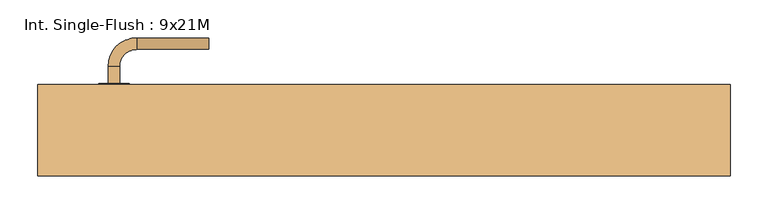
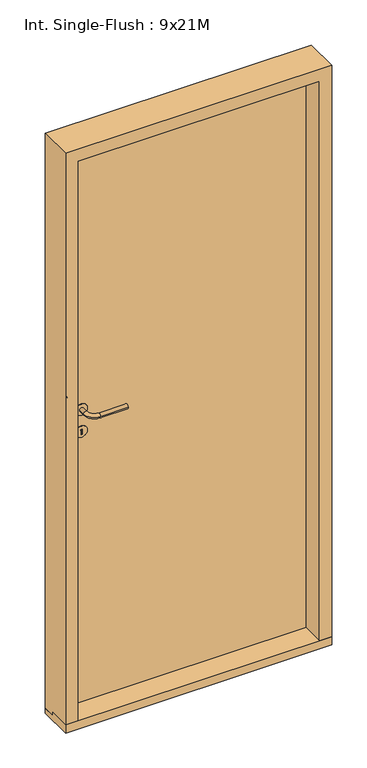
"""IFC4 building model written with IfcOpenShell, lengths in millimetres: door geometry, Int. Single-Flush : 9x21M."""

from ifc_helpers import new_model, si_unit, point, frame, frame_2d, origin, place, context, project, spatial, polyline, circle_curve, ellipse_curve, trimmed, segment, composite_curve, outline, extrude, faceted_brep, source, transform, mapped, element, save
from ifc_brep_helpers import plane_surface, cylinder_surface, revolved_surface, advanced_brep


def int_single_flush_9x21m_be440b31(model_context):
    return source(origin(), model_context, "Body", "SolidModel", [
        extrude(outline(composite_curve([segment(trimmed(circle_curve(frame_2d((1090.0, -356.0)), 20.0), [point((1070.0, -356.0))], [point((1110.0, -356.0))], False, "CARTESIAN"), True, "CONTINUOUS"), segment(trimmed(circle_curve(frame_2d((1090.0, -356.0)), 20.0), [point((1110.0, -356.0))], [point((1070.0, -356.0))], False, "CARTESIAN"), True, "CONTINUOUS")], self_intersect=False)), frame((0.0, 60.0, 0.0), z_axis=(0.0, 1.0, 0.0), x_axis=(0.0, 0.0, 1.0)), (0.0, 0.0, 1.0), 2.0),
        advanced_brep(
        [(-363.5, 62.0, 1090.0), (-348.5, 62.0, 1090.0), (-363.5, 84.5, 1090.0), (-348.5, 84.5, 1090.0), (-326.0, 107.0, 1090.0), (-326.0, 122.0, 1090.0), (-231.0, 122.0, 1090.0), (-231.0, 107.0, 1090.0)],
        [
            (0, 1, circle_curve(frame((-356.0, 62.0, 1090.0), z_axis=(0.0, -1.0, 0.0), x_axis=(1.0, 0.0, 0.0)), 7.5)),
            (1, 0, circle_curve(frame((-356.0, 62.0, 1090.0), z_axis=(0.0, -1.0, 0.0), x_axis=(1.0, 0.0, 0.0)), 7.5)),
            (0, 2),
            (2, 3, circle_curve(frame((-356.0, 84.5, 1090.0), z_axis=(0.0, -1.0, 0.0), x_axis=(1.0, 0.0, 0.0)), 7.5)),
            (3, 1),
            (3, 2, circle_curve(frame((-356.0, 84.5, 1090.0), z_axis=(0.0, -1.0, 0.0), x_axis=(1.0, 0.0, 0.0)), 7.5)),
            (4, 3, circle_curve(frame((-326.0, 84.5, 1090.0), z_axis=(0.0, 0.0, 1.0), x_axis=(-1.0, 0.0, 0.0)), 22.5)),
            (2, 5, circle_curve(frame((-326.0, 84.5, 1090.0), z_axis=(0.0, 0.0, -1.0), x_axis=(-1.0, 0.0, 0.0)), 37.5)),
            (5, 4, circle_curve(frame((-326.0, 114.5, 1090.0), z_axis=(-1.0, 0.0, 0.0), x_axis=(0.0, -1.0, 0.0)), 7.5)),
            (4, 5, circle_curve(frame((-326.0, 114.5, 1090.0), z_axis=(-1.0, 0.0, 0.0), x_axis=(0.0, -1.0, 0.0)), 7.5)),
            (5, 6),
            (6, 7, circle_curve(frame((-231.0, 114.5, 1090.0), z_axis=(-1.0, 0.0, 0.0), x_axis=(0.0, -1.0, 0.0)), 7.5)),
            (7, 4),
            (7, 6, circle_curve(frame((-231.0, 114.5, 1090.0), z_axis=(-1.0, 0.0, 0.0), x_axis=(0.0, -1.0, 0.0)), 7.5)),
        ],
        [
            plane_surface(frame((-356.0, 62.0, 1090.0), z_axis=(0.0, -1.0, 0.0), x_axis=(0.0, 0.0, -1.0))),
            cylinder_surface(frame((-356.0, 62.0, 1090.0), z_axis=(0.0, -1.0, 0.0), x_axis=(1.0, 0.0, 0.0)), 7.5),
            revolved_surface(trimmed(ellipse_curve(frame((-356.0, 84.5, 1090.0), z_axis=(0.0, -1.0, 0.0), x_axis=(1.0, 0.0, 0.0)), 7.5, 7.5), [point((-363.5, 84.5, 1090.0))], [point((-348.5, 84.5, 1090.0))], True, "CARTESIAN"), (-326.0, 84.5, 1090.0), (0.0, 0.0, -1.0)),
            revolved_surface(trimmed(ellipse_curve(frame((-356.0, 84.5, 1090.0), z_axis=(0.0, -1.0, 0.0), x_axis=(1.0, 0.0, 0.0)), 7.5, 7.5), [point((-348.5, 84.5, 1090.0))], [point((-363.5, 84.5, 1090.0))], True, "CARTESIAN"), (-326.0, 84.5, 1090.0), (0.0, 0.0, -1.0)),
            cylinder_surface(frame((-326.0, 114.5, 1090.0), z_axis=(-1.0, 0.0, 0.0), x_axis=(0.0, -1.0, 0.0)), 7.5),
            plane_surface(frame((-231.0, 114.5, 1090.0), z_axis=(1.0, 0.0, 0.0), x_axis=(0.0, 0.0, -1.0))),
        ],
        [
            (0, [[1, 2]]),
            (1, [[-1, 3, 4, 5]]),
            (1, [[-2, -5, 6, -3]]),
            (2, [[7, -4, 8, 9]]),
            (3, [[-8, -6, -7, 10]]),
            (4, [[-9, 11, 12, 13]]),
            (4, [[-10, -13, 14, -11]]),
            (5, [[-14, -12]]),
        ],
    ),
        extrude(outline(composite_curve([segment(trimmed(circle_curve(frame_2d((1010.0, -356.0)), 20.0), [point((990.0, -356.0))], [point((1030.0, -356.0))], False, "CARTESIAN"), True, "CONTINUOUS"), segment(trimmed(circle_curve(frame_2d((1010.0, -356.0)), 20.0), [point((1030.0, -356.0))], [point((990.0, -356.0))], False, "CARTESIAN"), True, "CONTINUOUS")], self_intersect=False), holes=[composite_curve([segment(trimmed(circle_curve(frame_2d((1015.0, -356.0)), 3.0), [point((1012.4019238, -357.5))], [point((1012.4019238, -354.5))], True, "CARTESIAN"), True, "CONTINUOUS"), segment(polyline([(1012.4019238, -354.5), (1000.0, -354.5), (1000.0, -357.5), (1012.4019238, -357.5)]), True, "CONTINUOUS")], self_intersect=False)]), frame((0.0, 60.0, 0.0), z_axis=(0.0, 1.0, 0.0), x_axis=(0.0, 0.0, 1.0)), (0.0, 0.0, 1.0), 2.0),
        extrude(outline(composite_curve([segment(trimmed(circle_curve(frame_2d((1090.0, -356.0)), 20.0), [point((1070.0, -356.0))], [point((1110.0, -356.0))], False, "CARTESIAN"), True, "CONTINUOUS"), segment(trimmed(circle_curve(frame_2d((1090.0, -356.0)), 20.0), [point((1110.0, -356.0))], [point((1070.0, -356.0))], False, "CARTESIAN"), True, "CONTINUOUS")], self_intersect=False)), frame((0.0, 18.0, 0.0), z_axis=(0.0, 1.0, 0.0), x_axis=(0.0, 0.0, 1.0)), (0.0, 0.0, 1.0), 2.0),
        advanced_brep(
        [(-363.5, 18.0, 1090.0), (-348.5, 18.0, 1090.0), (-348.5, -4.5, 1090.0), (-363.5, -4.5, 1090.0), (-326.0, -27.0, 1090.0), (-326.0, -42.0, 1090.0), (-231.0, -27.0, 1090.0), (-231.0, -42.0, 1090.0)],
        [
            (0, 1, circle_curve(frame((-356.0, 18.0, 1090.0), z_axis=(0.0, 1.0, 0.0), x_axis=(1.0, 0.0, 0.0)), 7.5)),
            (1, 0, circle_curve(frame((-356.0, 18.0, 1090.0), z_axis=(0.0, 1.0, 0.0), x_axis=(1.0, 0.0, 0.0)), 7.5)),
            (1, 2),
            (2, 3, circle_curve(frame((-356.0, -4.5, 1090.0), z_axis=(0.0, 1.0, 0.0), x_axis=(1.0, 0.0, 0.0)), 7.5)),
            (3, 0),
            (3, 2, circle_curve(frame((-356.0, -4.5, 1090.0), z_axis=(0.0, 1.0, 0.0), x_axis=(1.0, 0.0, 0.0)), 7.5)),
            (4, 5, circle_curve(frame((-326.0, -34.5, 1090.0), z_axis=(-1.0, 0.0, 0.0), x_axis=(0.0, 1.0, 0.0)), 7.5)),
            (5, 3, circle_curve(frame((-326.0, -4.5, 1090.0), z_axis=(0.0, 0.0, -1.0), x_axis=(-1.0, 0.0, 0.0)), 37.5)),
            (2, 4, circle_curve(frame((-326.0, -4.5, 1090.0), z_axis=(0.0, 0.0, 1.0), x_axis=(-1.0, 0.0, 0.0)), 22.5)),
            (5, 4, circle_curve(frame((-326.0, -34.5, 1090.0), z_axis=(-1.0, 0.0, 0.0), x_axis=(0.0, 1.0, 0.0)), 7.5)),
            (4, 6),
            (6, 7, circle_curve(frame((-231.0, -34.5, 1090.0), z_axis=(-1.0, 0.0, 0.0), x_axis=(0.0, 1.0, 0.0)), 7.5)),
            (7, 5),
            (7, 6, circle_curve(frame((-231.0, -34.5, 1090.0), z_axis=(-1.0, 0.0, 0.0), x_axis=(0.0, 1.0, 0.0)), 7.5)),
        ],
        [
            plane_surface(frame((-356.0, 18.0, 1090.0), z_axis=(0.0, 1.0, 0.0), x_axis=(0.0, 0.0, -1.0))),
            cylinder_surface(frame((-356.0, 18.0, 1090.0), z_axis=(0.0, 1.0, 0.0), x_axis=(1.0, 0.0, 0.0)), 7.5),
            revolved_surface(trimmed(ellipse_curve(frame((-356.0, -4.5, 1090.0), z_axis=(0.0, -1.0, 0.0), x_axis=(1.0, 0.0, 0.0)), 7.5, 7.5), [point((-363.5, -4.5, 1090.0))], [point((-348.5, -4.5, 1090.0))], True, "CARTESIAN"), (-326.0, -4.5, 1090.0), (0.0, 0.0, -1.0)),
            revolved_surface(trimmed(ellipse_curve(frame((-356.0, -4.5, 1090.0), z_axis=(0.0, -1.0, 0.0), x_axis=(1.0, 0.0, 0.0)), 7.5, 7.5), [point((-348.5, -4.5, 1090.0))], [point((-363.5, -4.5, 1090.0))], True, "CARTESIAN"), (-326.0, -4.5, 1090.0), (0.0, 0.0, -1.0)),
            cylinder_surface(frame((-326.0, -34.5, 1090.0), z_axis=(-1.0, 0.0, 0.0), x_axis=(0.0, 1.0, 0.0)), 7.5),
            plane_surface(frame((-231.0, -34.5, 1090.0), z_axis=(1.0, 0.0, 0.0), x_axis=(0.0, 0.0, -1.0))),
        ],
        [
            (0, [[1, 2]]),
            (1, [[3, 4, 5, -2]]),
            (1, [[-5, 6, -3, -1]]),
            (2, [[7, 8, -4, 9]]),
            (3, [[10, -9, -6, -8]]),
            (4, [[11, 12, 13, -7]]),
            (4, [[-13, 14, -11, -10]]),
            (5, [[-12, -14]]),
        ],
    ),
        extrude(outline(composite_curve([segment(trimmed(circle_curve(frame_2d((1010.0, -356.0)), 20.0), [point((990.0, -356.0))], [point((1030.0, -356.0))], False, "CARTESIAN"), True, "CONTINUOUS"), segment(trimmed(circle_curve(frame_2d((1010.0, -356.0)), 20.0), [point((1030.0, -356.0))], [point((990.0, -356.0))], False, "CARTESIAN"), True, "CONTINUOUS")], self_intersect=False), holes=[composite_curve([segment(trimmed(circle_curve(frame_2d((1015.0, -356.0)), 3.0), [point((1012.4019238, -357.5))], [point((1012.4019238, -354.5))], True, "CARTESIAN"), True, "CONTINUOUS"), segment(polyline([(1012.4019238, -354.5), (1000.0, -354.5), (1000.0, -357.5), (1012.4019238, -357.5)]), True, "CONTINUOUS")], self_intersect=False)]), frame((0.0, 18.0, 0.0), z_axis=(0.0, 1.0, 0.0), x_axis=(0.0, 0.0, 1.0)), (0.0, 0.0, 1.0), 2.0),
        extrude(outline(polyline([(426.0, 20.0), (-426.0, 20.0), (-426.0, 60.0), (426.0, 60.0), (426.0, 20.0)])), frame((0.0, 0.0, 18.0), z_axis=(0.0, 0.0, 1.0), x_axis=(1.0, 0.0, 0.0)), (0.0, 0.0, 1.0), 2052.0),
        faceted_brep([(-426.0, 20.0, 2070.0), (426.0, 20.0, 2070.0), (426.0, 20.0, 30.0), (414.0, 20.0, 30.0), (414.0, 20.0, 2058.0), (-414.0, 20.0, 2058.0), (-414.0, 20.0, 30.0), (-426.0, 20.0, 30.0), (-426.0, 60.0, 2070.0), (-426.0, 20.0, 18.0), (-426.0, 60.0, 18.0), (-456.0, 20.0, 30.0), (-456.0, 20.0, 18.0), (456.0, 20.0, 30.0), (426.0, 20.0, 18.0), (456.0, 20.0, 18.0), (-456.0, 60.0, 18.0), (426.0, 60.0, 18.0), (456.0, 60.0, 18.0), (-456.0, 60.0, 2100.0), (456.0, 60.0, 2100.0), (426.0, 60.0, 2070.0), (-414.0, -60.0, 30.0), (-456.0, -60.0, 30.0), (456.0, -60.0, 30.0), (414.0, -60.0, 30.0), (414.0, -60.0, 2058.0), (-414.0, -60.0, 2058.0), (456.0, -60.0, 2100.0), (-456.0, -60.0, 2100.0)], [[[0, 1, 2, 3, 4, 5, 6, 7]], [[8, 0, 7, 9, 10]], [[7, 11, 12, 9]], [[13, 2, 14, 15]], [[9, 12, 16, 10]], [[15, 14, 17, 18]], [[19, 20, 18, 17, 21, 8, 10, 16]], [[1, 21, 17, 14, 2]], [[11, 7, 6, 22, 23]], [[2, 13, 24, 25, 3]], [[26, 4, 3, 25]], [[5, 27, 22, 6]], [[27, 26, 25, 24, 28, 29, 23, 22]], [[20, 28, 24, 13, 15, 18]], [[29, 19, 16, 12, 11, 23]], [[0, 8, 21, 1]], [[5, 4, 26, 27]], [[29, 28, 20, 19]]]),
        extrude(outline(polyline([(20.0, 30.0), (20.0, 18.0), (60.0, 18.0), (60.0, 0.0), (-60.0, 0.0), (-60.0, 30.0), (20.0, 30.0)])), frame((-456.0, 0.0, 0.0), z_axis=(1.0, 0.0, 0.0), x_axis=(0.0, 1.0, 0.0)), (0.0, 0.0, 1.0), 912.0),
    ])


if __name__ == "__main__":
    model = new_model("IFC4")
    model_context = context("Model", 3, world=origin())
    ifc_project = project(units=[si_unit("LENGTHUNIT", "METRE", prefix="MILLI")], contexts=[model_context])
    site = spatial("IfcSite", under=ifc_project)
    building = spatial("IfcBuilding", under=site)
    placement = place(None, origin())
    int_single_flush_9x21m_shape = int_single_flush_9x21m_be440b31(model_context)
    element("IfcDoor", 1, ObjectType="Int. Single-Flush : 9x21M", at=placement, inside=building, context=model_context, shape_type="MappedRepresentation", body=[
        mapped(int_single_flush_9x21m_shape, transform((0.0, 0.0, 0.0), x_axis=(1.0, 0.0, 0.0), y_axis=(0.0, 1.0, 0.0), z_axis=(0.0, 0.0, 1.0))),
    ])
    save(model, "model.ifc")

# Revit data of these elements
# Type "Int. Single-Flush : 9x21M"
#   Type Mark = "53"
#   Sound Rating = ""
#   Hinge Side [instance default] = ""
#   Creator Build [instance default] = "2017.0301.0"
#   Creator Organization [instance default] = "© Danish Educational Content"
#   Creator Name [instance default] = "© Erik Falck Jørgensen"
#   Analytic Construction = "<None>"
#   length#3 = 18 mm
#   length#2 = 42 mm
#   length#1 = 0 mm
#   length#4 = 912 mm
#   Thickness = 40 mm
#   Seal Width = 12 mm
#   Rough Width = 912 mm
#   Rough Height = 2100 mm
#   Rabbet Width = 12 mm
#   Rabbet Depth = 40 mm
#   Interior Distance [instance default] = 0 mm
#   Height = 2088 mm
#   Width = 888 mm
#   Handle From Side = 100 mm
#   Handle From Bottom = 1090 mm
#   Exterior Direction [instance default] = 0.00°
#   Case Depth [instance default] = 200 mm
#   Case Width = 30 mm
#   Exterior Distance [instance default] = 0 mm
#   Threshold = yes
#   Sealing = no
#   Hinging = yes
#   Wall Closure = 1
#   Door Panel = no
#   Panel = none
#   Handle Finish = none
#   Handle = element 510752
#   Case/Transom = none
#   Function = (empty or 0)
#   Assembly Code = ""
# Element 1 (IfcDoor, "Int. Single-Flush : 9x21M")
#   Case Depth = 120 mm
#   Materials on its faces: "Stainless Steel, Polished", "Default Frame/Mullion (Interior/Exterior)", "Default Door Panel (Exterior/Interior)"
# Materials
#   "Stainless Steel, Polished": class "Metal", colour RGB 180 180 180, transparency 0, Description = "Rustfri stål, poleret", Cost = 0
#   "Default Frame/Mullion (Interior/Exterior)": class "Generic", colour RGB 205 205 205, transparency 0, Description = "Udefineret karm/ramme materiale", Cost = 0
#   "Default Door Panel (Exterior/Interior)": class "Generic", colour RGB 205 205 205, transparency 0, Description = "Udefineret dørplade materiale", Cost = 0
